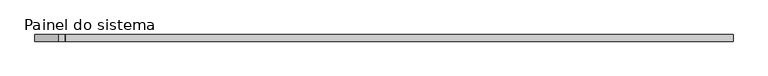
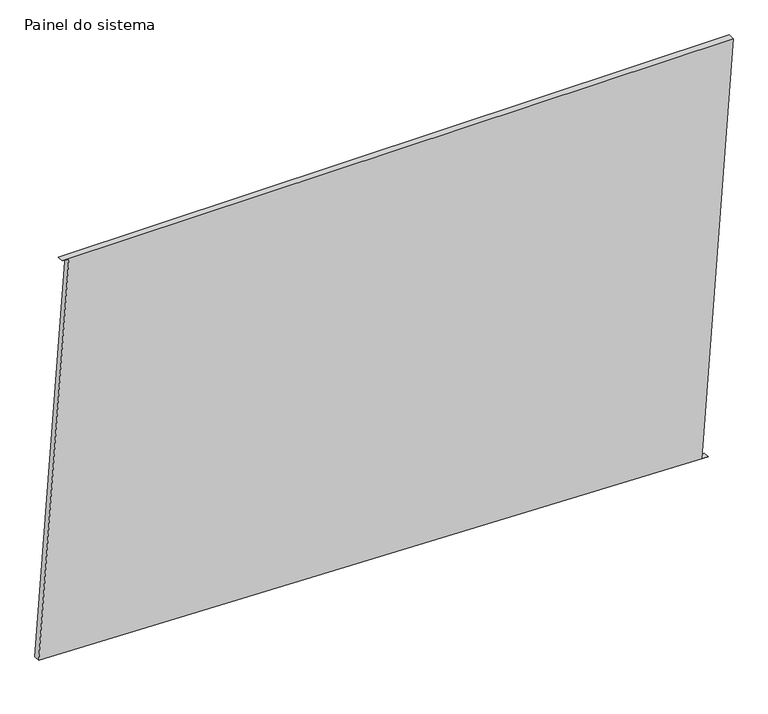
"""IFC4 building model written with IfcOpenShell, lengths in millimetres: plate geometry, Painel do sistema : Envidraçado."""

from ifc_helpers import new_model, si_unit, frame, origin, place, context, project, spatial, polyline, outline, extrude, source, transform, mapped, element, save


def painel_do_sistema_7d677d63(model_context):
    return source(origin(), model_context, "Body", "SweptSolid", [
        extrude(outline(polyline([(0.0, 1226.9411179), (1.8159485, 1202.0071585), (1650.5962686, 1322.088373), (1650.5962686, -1232.2882683), (1648.7803201, -1207.3543089), (73.4192812, -1322.088373), (0.0, 1226.9411179)])), frame((0.0, 24.5, 0.0), z_axis=(0.0, 1.0, 0.0), x_axis=(0.0, 0.0, 1.0)), (0.0, 0.0, 1.0), 25.0),
    ])


if __name__ == "__main__":
    model = new_model("IFC4")
    model_context = context("Model", 3, world=origin())
    ifc_project = project(units=[si_unit("LENGTHUNIT", "METRE", prefix="MILLI")], contexts=[model_context])
    site = spatial("IfcSite", under=ifc_project)
    building = spatial("IfcBuilding", under=site)
    placement = place(None, origin())
    painel_do_sistema_shape = painel_do_sistema_7d677d63(model_context)
    element("IfcPlate", 1, ObjectType="Painel do sistema : Envidraçado", at=placement, inside=building, context=model_context, shape_type="MappedRepresentation", body=[
        mapped(painel_do_sistema_shape, transform((0.0, 0.0, 0.0), x_axis=(1.0, 0.0, 0.0), y_axis=(0.0, 1.0, 0.0), z_axis=(0.0, 0.0, 1.0))),
    ])
    save(model, "model.ifc")

# Revit data of these elements
# Type "Painel do sistema : Envidraçado"
#   Construction Type Id = "GSP4R"
#   Analytic Construction = "Vidraça única Pilkington 1/8 pol"
#   Visual Light Transmittance = 0.9
#   Solar Heat Gain Coefficient = 0.86
#   Heat Transfer Coefficient (U) = 6.7069 W/(m²·K)
# Element 1 (IfcPlate, "Painel do sistema : Envidraçado")
#   Materials on its faces: "Vidro"
# Materials
#   "Vidro": class "Vidro", colour RGB 0 128 192, transparency 0.9, Description = "Vidro de sílica", Cost = 0
